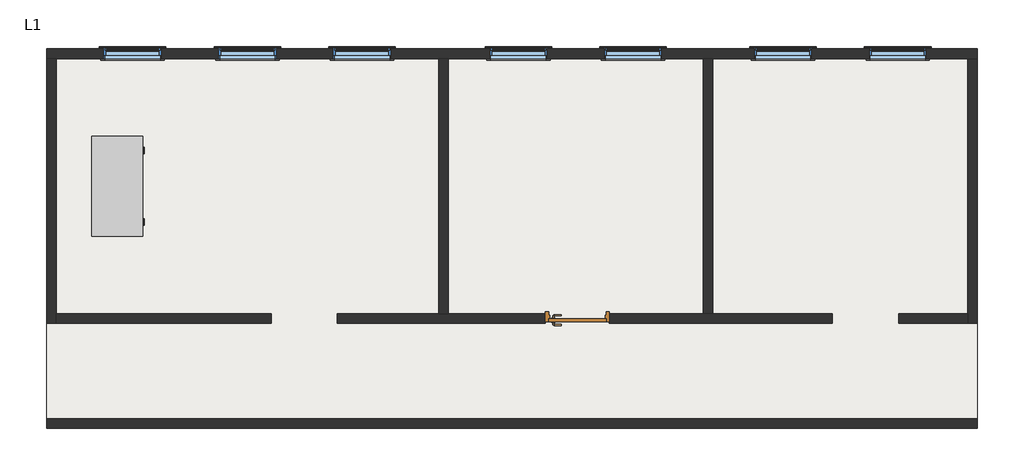
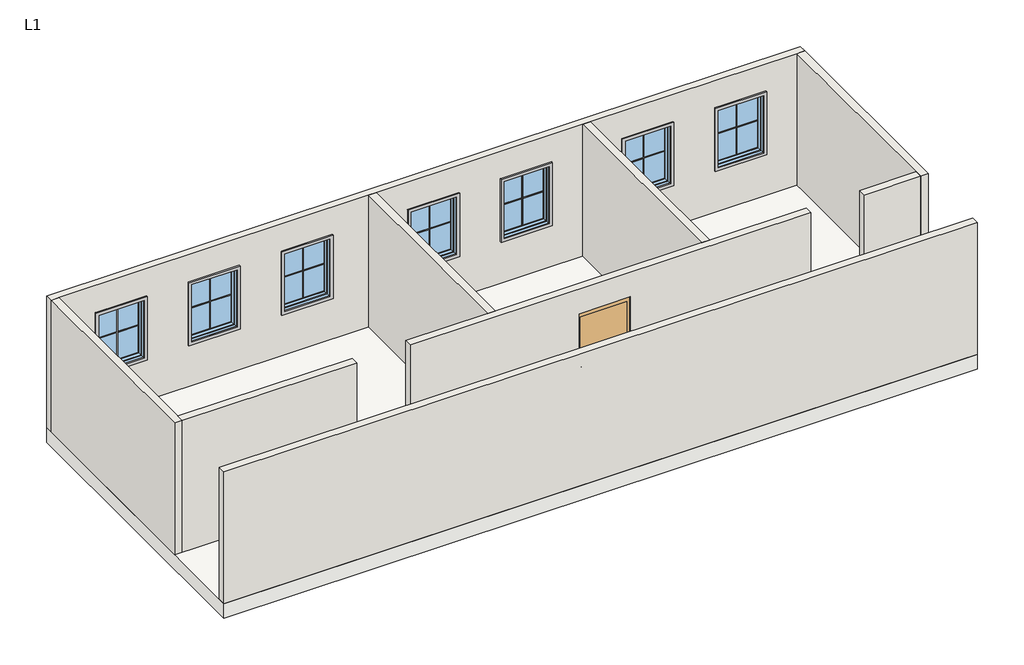
# One storey: 21 proxies, 9 walls, 7 windows, 1 door, 1 furniture element, 1 slab.
"""IFC4 building model written with IfcOpenShell, lengths in millimetres."""

import ifcopenshell
import ifcopenshell.guid

model = None  # the IFC model being written
_history = None  # IfcOwnerHistory: only IFC2X3 demands one
_inside = {}  # id of a spatial element -> (the spatial element, [elements in it])
_under = {}  # id of a project, library or spatial element -> (it, [spatial elements below it])
_declared = {}  # id of a project -> (the project, [libraries it declares])
_typed = {}  # id of a type object -> (the type object, [elements of that type])
_made_of = {}  # id of a material, layer set ... -> (it, [elements and type objects made of it])


def new_model(schema):
    """Start an empty IFC model of exactly this schema.

    Asked for "IFC4X3", IfcOpenShell would pick the latest addendum, in which some entities
    have other attributes; the version numbers below select the first issue.
    IFC2X3 requires an IfcOwnerHistory on every rooted entity: one is made here for all.
    """
    global model, _history
    if schema == "IFC4X3":
        model = ifcopenshell.file(schema_version=(4, 3, 0, 0))
    else:
        model = ifcopenshell.file(schema=schema)
    _inside.clear()
    _under.clear()
    _declared.clear()
    _typed.clear()
    _made_of.clear()
    _history = None
    if model.schema == "IFC2X3":
        org = make("IfcOrganization", Name="unknown")
        user = make(
            "IfcPersonAndOrganization",
            ThePerson=make("IfcPerson", FamilyName="unknown"),
            TheOrganization=org,
        )
        app = make(
            "IfcApplication",
            ApplicationDeveloper=org,
            Version="unknown",
            ApplicationFullName="unknown",
            ApplicationIdentifier="unknown",
        )
        _history = make(
            "IfcOwnerHistory",
            OwningUser=user,
            OwningApplication=app,
            ChangeAction="ADDED",
            CreationDate=0,
        )
    return model


def make(cls, **values):
    """One entity of the class cls with the attributes given. An attribute that is None is left unset."""
    return model.create_entity(
        cls, **{name: value for name, value in values.items() if value is not None}
    )


def rooted(cls, **values):
    """An entity with a GlobalId (a new one), such as an element, a storey or a relation."""
    return make(cls, GlobalId=ifcopenshell.guid.new(), OwnerHistory=_history, **values)


def si_unit(unit_type, name, prefix=None):
    """IfcSIUnit, for example si_unit("LENGTHUNIT", "METRE", prefix="MILLI")."""
    return make("IfcSIUnit", UnitType=unit_type, Prefix=prefix, Name=name)


def assignment(units):
    """IfcUnitAssignment: the units of a project."""
    return None if units is None else make("IfcUnitAssignment", Units=units)


def point(xyz):
    """IfcCartesianPoint."""
    return None if xyz is None else make("IfcCartesianPoint", Coordinates=xyz)


def direction(xyz):
    """IfcDirection."""
    return None if xyz is None else make("IfcDirection", DirectionRatios=xyz)


def frame(location, z_axis=None, x_axis=None):
    """IfcAxis2Placement3D, a coordinate frame: its origin and axes. An axis left out is left unset."""
    return make(
        "IfcAxis2Placement3D",
        Location=point(location),
        Axis=direction(z_axis),
        RefDirection=direction(x_axis),
    )


def frame_2d(location, x_axis=None):
    """IfcAxis2Placement2D, a coordinate frame in the plane: its origin and x axis."""
    return make(
        "IfcAxis2Placement2D", Location=point(location), RefDirection=direction(x_axis)
    )


def origin():
    """The frame at (0, 0, 0) with its axes left unset."""
    return frame((0.0, 0.0, 0.0))


def origin_with_axes():
    """The frame at (0, 0, 0) with the z axis (0, 0, 1) and the x axis (1, 0, 0) written out."""
    return frame((0.0, 0.0, 0.0), z_axis=(0.0, 0.0, 1.0), x_axis=(1.0, 0.0, 0.0))


def place(relative_to, where):
    """IfcLocalPlacement: puts the frame where relative to a parent placement (None: the world)."""
    return make(
        "IfcLocalPlacement", PlacementRelTo=relative_to, RelativePlacement=where
    )


def context(
    kind, dimensions, precision=None, world=None, true_north=None, identifier=None
):
    """IfcGeometricRepresentationContext, for example the 3D "Model" context."""
    return make(
        "IfcGeometricRepresentationContext",
        ContextIdentifier=identifier,
        ContextType=kind,
        CoordinateSpaceDimension=dimensions,
        Precision=precision,
        WorldCoordinateSystem=world,
        TrueNorth=true_north,
    )


def project(units=None, contexts=None):
    """IfcProject with its units and contexts."""
    return rooted(
        "IfcProject",
        Name="project",
        RepresentationContexts=contexts,
        UnitsInContext=assignment(units),
    )


def spatial(cls, under=None, at=None, **own):
    """A site, building, storey or space (cls), placed at a placement, below another one or the project."""
    s = rooted(cls, ObjectPlacement=at, **own)
    if under is not None:
        _under.setdefault(under.id(), (under, []))[1].append(s)
    return s


def polyline(points):
    """IfcPolyline through the points."""
    return make("IfcPolyline", Points=[point(p) for p in points])


def circle_curve(where, radius):
    """IfcCircle in the frame where."""
    return make("IfcCircle", Position=where, Radius=radius)


def ellipse_curve(where, semi_axis1, semi_axis2):
    """IfcEllipse in the frame where."""
    return make(
        "IfcEllipse", Position=where, SemiAxis1=semi_axis1, SemiAxis2=semi_axis2
    )


def trimmed(basis, trim1, trim2, sense, master):
    """IfcTrimmedCurve: the piece of a basis curve between two trims."""
    return make(
        "IfcTrimmedCurve",
        BasisCurve=basis,
        Trim1=trim1,
        Trim2=trim2,
        SenseAgreement=sense,
        MasterRepresentation=master,
    )


def segment(curve, same_sense, transition):
    """IfcCompositeCurveSegment."""
    return make(
        "IfcCompositeCurveSegment",
        Transition=transition,
        SameSense=same_sense,
        ParentCurve=curve,
    )


def composite_curve(segments, self_intersect=None):
    """IfcCompositeCurve: segments joined end to end."""
    return make("IfcCompositeCurve", Segments=segments, SelfIntersect=self_intersect)


def outline(outer, holes=None, kind="AREA"):
    """IfcArbitraryClosedProfileDef: a profile drawn as a closed curve; with holes, ...WithVoids."""
    if holes is None:
        return make("IfcArbitraryClosedProfileDef", ProfileType=kind, OuterCurve=outer)
    return make(
        "IfcArbitraryProfileDefWithVoids",
        ProfileType=kind,
        OuterCurve=outer,
        InnerCurves=holes,
    )


def extrude(swept, where, along, depth):
    """IfcExtrudedAreaSolid: the profile swept, set in the frame where, extruded along a direction by depth."""
    return make(
        "IfcExtrudedAreaSolid",
        SweptArea=swept,
        Position=where,
        ExtrudedDirection=direction(along),
        Depth=depth,
    )


def faces_of(points, faces, orient=None, outer=None):
    """IfcFace entities. A face is a list of loops; a loop is a list of indices into points, from 0.

    orient and outer hold one flag for each loop. By default every Orientation is true, the
    first loop of a face is its IfcFaceOuterBound and the others are IfcFaceBound.
    """
    made = []
    for i, loops in enumerate(faces):
        bounds = []
        for j, loop in enumerate(loops):
            is_outer = j == 0 if outer is None else outer[i][j]
            bounds.append(
                make(
                    "IfcFaceOuterBound" if is_outer else "IfcFaceBound",
                    Bound=make("IfcPolyLoop", Polygon=[points[k] for k in loop]),
                    Orientation=True if orient is None else orient[i][j],
                )
            )
        made.append(make("IfcFace", Bounds=bounds))
    return made


def faceted_brep(points, faces, orient=None, outer=None, voids=None):
    """IfcFacetedBrep: a solid bounded by flat faces; with voids (closed shells), ...WithVoids."""
    shared = [point(p) for p in points]
    hull = make("IfcClosedShell", CfsFaces=faces_of(shared, faces, orient, outer))
    if voids is None:
        return make("IfcFacetedBrep", Outer=hull)
    return make(
        "IfcFacetedBrepWithVoids",
        Outer=hull,
        Voids=[
            make(cls, CfsFaces=faces_of(shared, fs, o, b)) for cls, fs, o, b in voids
        ],
    )


def shape(context_of_items, identifier, shape_type, items):
    """IfcShapeRepresentation: the items that make up one representation, for example the "Body"."""
    return make(
        "IfcShapeRepresentation",
        ContextOfItems=context_of_items,
        RepresentationIdentifier=identifier,
        RepresentationType=shape_type,
        Items=items,
    )


def source(mapping_origin, context_of_items, identifier, shape_type, items):
    """IfcRepresentationMap: a shape defined once, which mapped items show again and again."""
    return make(
        "IfcRepresentationMap",
        MappingOrigin=mapping_origin,
        MappedRepresentation=shape(context_of_items, identifier, shape_type, items),
    )


def transform(
    local_origin,
    x_axis=None,
    y_axis=None,
    z_axis=None,
    scale=None,
    scale2=None,
    scale3=None,
    uniform=True,
):
    """IfcCartesianTransformationOperator3D, or its non-uniform kind. x_axis, y_axis, z_axis: its Axis1, 2, 3."""
    if uniform:
        return make(
            "IfcCartesianTransformationOperator3D",
            Axis1=direction(x_axis),
            Axis2=direction(y_axis),
            LocalOrigin=point(local_origin),
            Scale=scale,
            Axis3=direction(z_axis),
        )
    return make(
        "IfcCartesianTransformationOperator3DnonUniform",
        Axis1=direction(x_axis),
        Axis2=direction(y_axis),
        LocalOrigin=point(local_origin),
        Scale=scale,
        Axis3=direction(z_axis),
        Scale2=scale2,
        Scale3=scale3,
    )


def mapped(mapping_source, mapping_target):
    """IfcMappedItem: shows the shape of a source again, moved by a transform."""
    return make(
        "IfcMappedItem", MappingSource=mapping_source, MappingTarget=mapping_target
    )


def made_of(thing, what):
    """Note that an element or type object is made of a material, layer set ...; save() writes the relation."""
    if what is not None:
        _made_of.setdefault(what.id(), (what, []))[1].append(thing)
    return thing


def element(
    cls,
    number,
    at=None,
    inside=None,
    cuts=None,
    type_object=None,
    material=None,
    context=None,
    identifier="Body",
    shape_type=None,
    held_by="IfcProductDefinitionShape",
    body=None,
    shapes=None,
    **own,
):
    """One element of the class cls, such as IfcWall. Its Tag is "e" and its number.

    at: its placement. inside: the storey or other place that contains it. cuts: it is an
    opening in that element (IfcRelVoidsElement). A single representation is given by context,
    identifier, shape_type and body (its items); several are given by shapes. held_by: the class
    of the entity that holds the representations. save() writes the other relations.
    """
    e = rooted(cls, Tag="e%d" % number, ObjectPlacement=at, **own)
    if body is not None:
        shapes = [shape(context, identifier, shape_type, body)]
    if shapes is not None:
        e.Representation = make(held_by, Representations=shapes)
    if inside is not None:
        _inside.setdefault(inside.id(), (inside, []))[1].append(e)
    if cuts is not None:
        rooted(
            "IfcRelVoidsElement", RelatingBuildingElement=cuts, RelatedOpeningElement=e
        )
    if type_object is not None:
        _typed.setdefault(type_object.id(), (type_object, []))[1].append(e)
    return made_of(e, material)


def aggregate(whole, parts):
    """IfcRelAggregates: a whole, such as a stair, and the parts it consists of."""
    return rooted("IfcRelAggregates", RelatingObject=whole, RelatedObjects=parts)


def save(model, path):
    """Write the relations noted so far, then the file.

    IfcRelAggregates (storeys below a building ...), IfcRelContainedInSpatialStructure (elements
    in a storey), IfcRelDefinesByType, IfcRelAssociatesMaterial and IfcRelDeclares: one each for
    every whole, place, type object, material and project.
    """
    for whole, parts in _under.values():
        aggregate(whole, parts)
    for where, things in _inside.values():
        rooted(
            "IfcRelContainedInSpatialStructure",
            RelatedElements=things,
            RelatingStructure=where,
        )
    for kind, things in _typed.values():
        rooted("IfcRelDefinesByType", RelatedObjects=things, RelatingType=kind)
    for what, things in _made_of.values():
        rooted("IfcRelAssociatesMaterial", RelatedObjects=things, RelatingMaterial=what)
    for by, libraries in _declared.values():
        rooted("IfcRelDeclares", RelatingContext=by, RelatedDefinitions=libraries)
    model.write(path)


def plane_surface(at):
    """IfcPlane: the flat surface through the origin of the frame at, square to its z axis."""
    return make("IfcPlane", Position=at)


def cylinder_surface(at, radius):
    """IfcCylindricalSurface: all points at the distance radius from the z axis of the frame at."""
    return make("IfcCylindricalSurface", Position=at, Radius=radius)


def revolved_surface(curve, axis_point, axis_direction):
    """IfcSurfaceOfRevolution: the curve turned about the line through axis_point along axis_direction."""
    return make(
        "IfcSurfaceOfRevolution",
        SweptCurve=make("IfcArbitraryOpenProfileDef", ProfileType="CURVE", Curve=curve),
        AxisPosition=make("IfcAxis1Placement", Location=point(axis_point), Axis=direction(axis_direction)),
    )


def advanced_brep(points, edges, surfaces, faces):
    """IfcAdvancedBrep: a solid bounded by faces that lie on surfaces and meet in shared edges.

    An edge is (start, end): straight between two places in points (the first is 0);
    or (start, end, curve); or (start, end, curve, False) where it runs against its curve.
    A face is (place in surfaces, loops), or (place, loops, False) where it looks against
    its surface's normal. A loop lists edges by number (the first is 1), with a minus sign
    where the edge is run from its end to its start. The first loop is the outer one.
    """
    corners = [point(p) for p in points]
    vertices = [make("IfcVertexPoint", VertexGeometry=c) for c in corners]
    made = []
    for start, end, *more in edges:
        made.append(
            make(
                "IfcEdgeCurve",
                EdgeStart=vertices[start],
                EdgeEnd=vertices[end],
                EdgeGeometry=more[0] if more else make("IfcPolyline", Points=[corners[start], corners[end]]),
                SameSense=more[1] if len(more) > 1 else True,
            )
        )
    hull = []
    for where, loops, *sense in faces:
        bounds = []
        for j, loop in enumerate(loops):
            ring = [make("IfcOrientedEdge", EdgeElement=made[abs(k) - 1], Orientation=k > 0) for k in loop]
            bounds.append(
                make(
                    "IfcFaceOuterBound" if j == 0 else "IfcFaceBound",
                    Bound=make("IfcEdgeLoop", EdgeList=ring),
                    Orientation=True,
                )
            )
        hull.append(make("IfcAdvancedFace", Bounds=bounds, FaceSurface=surfaces[where], SameSense=sense[0] if sense else True))
    return make("IfcAdvancedBrep", Outer=make("IfcClosedShell", CfsFaces=hull))


def m_muntin_pattern_2x2_m_muntin_pattern_2x2_ad852c99(model_context):
    return source(origin(), model_context, "Body", "SweptSolid", [
        extrude(outline(polyline([(568.25, -6.35), (568.25, -411.9), (555.55, -411.9), (555.55, -6.35), (0.0, -6.35), (0.0, 6.35), (555.55, 6.35), (555.55, 411.9), (568.25, 411.9), (568.25, 6.35), (1123.8, 6.35), (1123.8, -6.35), (568.25, -6.35)])), frame((0.0, -22.225, 0.0), z_axis=(0.0, 1.0, 0.0), x_axis=(0.0, 0.0, 1.0)), (0.0, 0.0, 1.0), 12.7),
        extrude(outline(polyline([(568.25, -6.35), (568.25, -411.9), (555.55, -411.9), (555.55, -6.35), (0.0, -6.35), (0.0, 6.35), (555.55, 6.35), (555.55, 411.9), (568.25, 411.9), (568.25, 6.35), (1123.8, 6.35), (1123.8, -6.35), (568.25, -6.35)])), frame((0.0, 9.525, 0.0), z_axis=(0.0, 1.0, 0.0), x_axis=(0.0, 0.0, 1.0)), (0.0, 0.0, 1.0), 12.7),
    ])


def m_trim_window_exterior_flat_with_sill_71544b40(model_context):
    return source(origin(), model_context, "Body", "SweptSolid", [
        extrude(outline(polyline([(510.0, -1220.4323709), (510.0, -1280.4323709), (-510.0, -1280.4323709), (-510.0, -1220.4323709), (510.0, -1220.4323709)])), origin_with_axes(), (0.0, 0.0, 1.0), 19.05),
        extrude(outline(polyline([(-1230.0, 38.1), (-1202.4580645, 38.1), (-1200.0, 19.05), (-1200.0, 0.0), (-1220.4323709, 0.0), (-1220.4323709, 19.05), (-1230.0, 19.05), (-1230.0, 38.1)])), frame((-522.7, 0.0, 0.0), z_axis=(1.0, 0.0, 0.0), x_axis=(0.0, 1.0, 0.0)), (0.0, 0.0, 1.0), 1045.4),
        extrude(outline(polyline([(-510.0, 60.0), (510.0, 60.0), (510.0, -1200.0), (450.0, -1200.0), (450.0, 0.0), (-450.0, 0.0), (-450.0, -1200.0), (-510.0, -1200.0), (-510.0, 60.0)])), origin_with_axes(), (0.0, 0.0, 1.0), 19.05),
    ])


def m_trim_window_interior_flat_picture_frame_24fe8ef8(model_context):
    return source(origin(), model_context, "Body", "SweptSolid", [
        extrude(outline(polyline([(497.3, 47.3), (497.3, -1247.3), (-497.3, -1247.3), (-497.3, 47.3), (497.3, 47.3)]), holes=[polyline([(437.3, -12.7), (-437.3, -12.7), (-437.3, -1187.3), (437.3, -1187.3), (437.3, -12.7)])]), origin_with_axes(), (0.0, 0.0, 1.0), 30.0),
    ])


def m_door_passage_single_flush_900_x_2100mm_89322b7b(model_context):
    return source(origin(), model_context, "Body", "SolidModel", [
        advanced_brep(
        [(-384.990625, -3.35, 1000.0), (-364.990625, -3.35, 1000.0), (-384.990625, 26.65, 1000.0), (-364.990625, 26.65, 1000.0), (-359.990625, 31.65, 1000.0), (-359.990625, 51.65, 1000.0), (-254.990625, 51.65, 1000.0), (-254.990625, 31.65, 1000.0)],
        [
            (0, 1, circle_curve(frame((-374.990625, -3.35, 1000.0), z_axis=(0.0, -1.0, 0.0), x_axis=(1.0, 0.0, 0.0)), 10.0)),
            (1, 0, circle_curve(frame((-374.990625, -3.35, 1000.0), z_axis=(0.0, -1.0, 0.0), x_axis=(1.0, 0.0, 0.0)), 10.0)),
            (0, 2),
            (2, 3, circle_curve(frame((-374.990625, 26.65, 1000.0), z_axis=(0.0, -1.0, 0.0), x_axis=(1.0, 0.0, 0.0)), 10.0)),
            (3, 1),
            (3, 2, circle_curve(frame((-374.990625, 26.65, 1000.0), z_axis=(0.0, -1.0, 0.0), x_axis=(1.0, 0.0, 0.0)), 10.0)),
            (4, 3, circle_curve(frame((-359.990625, 26.65, 1000.0), z_axis=(0.0, 0.0, 1.0), x_axis=(-1.0, 0.0, 0.0)), 5.0)),
            (2, 5, circle_curve(frame((-359.990625, 26.65, 1000.0), z_axis=(0.0, 0.0, -1.0), x_axis=(-1.0, 0.0, 0.0)), 25.0)),
            (5, 4, circle_curve(frame((-359.990625, 41.65, 1000.0), z_axis=(-1.0, 0.0, 0.0), x_axis=(0.0, -1.0, 0.0)), 10.0)),
            (4, 5, circle_curve(frame((-359.990625, 41.65, 1000.0), z_axis=(-1.0, 0.0, 0.0), x_axis=(0.0, -1.0, 0.0)), 10.0)),
            (6, 7, circle_curve(frame((-254.990625, 41.65, 1000.0), z_axis=(1.0, 0.0, 0.0), x_axis=(0.0, -1.0, 0.0)), 10.0)),
            (7, 6, circle_curve(frame((-254.990625, 41.65, 1000.0), z_axis=(1.0, 0.0, 0.0), x_axis=(0.0, -1.0, 0.0)), 10.0)),
            (5, 6),
            (7, 4),
        ],
        [
            plane_surface(frame((-374.990625, -3.35, 1000.0), z_axis=(0.0, -1.0, 0.0), x_axis=(0.0, 0.0, 1.0))),
            cylinder_surface(frame((-374.990625, -3.35, 1000.0), z_axis=(0.0, -1.0, 0.0), x_axis=(1.0, 0.0, 0.0)), 10.0),
            revolved_surface(trimmed(ellipse_curve(frame((-374.990625, 26.65, 1000.0), z_axis=(0.0, -1.0, 0.0), x_axis=(1.0, 0.0, 0.0)), 10.0, 10.0), [point((-384.990625, 26.65, 1000.0))], [point((-364.990625, 26.65, 1000.0))], True, "CARTESIAN"), (-359.990625, 26.65, 1000.0), (0.0, 0.0, -1.0)),
            revolved_surface(trimmed(ellipse_curve(frame((-374.990625, 26.65, 1000.0), z_axis=(0.0, -1.0, 0.0), x_axis=(1.0, 0.0, 0.0)), 10.0, 10.0), [point((-364.990625, 26.65, 1000.0))], [point((-384.990625, 26.65, 1000.0))], True, "CARTESIAN"), (-359.990625, 26.65, 1000.0), (0.0, 0.0, -1.0)),
            plane_surface(frame((-254.990625, 41.65, 1000.0), z_axis=(1.0, 0.0, 0.0), x_axis=(0.0, 0.0, 1.0))),
            cylinder_surface(frame((-359.990625, 41.65, 1000.0), z_axis=(-1.0, 0.0, 0.0), x_axis=(0.0, -1.0, 0.0)), 10.0),
        ],
        [
            (0, [[1, 2]]),
            (1, [[-1, 3, 4, 5]]),
            (1, [[-2, -5, 6, -3]]),
            (2, [[7, -4, 8, 9]]),
            (3, [[-8, -6, -7, 10]]),
            (4, [[11, 12]]),
            (5, [[-9, 13, -12, 14]]),
            (5, [[-10, -14, -11, -13]]),
        ],
    ),
        extrude(outline(composite_curve([segment(trimmed(circle_curve(frame_2d((1000.0, -377.490625)), 30.0), [point((1000.0, -407.490625))], [point((1000.0, -347.490625))], False, "CARTESIAN"), True, "CONTINUOUS"), segment(trimmed(circle_curve(frame_2d((1000.0, -377.490625)), 30.0), [point((1000.0, -347.490625))], [point((1000.0, -407.490625))], False, "CARTESIAN"), True, "CONTINUOUS")], self_intersect=False)), frame((0.0, -11.35, 0.0), z_axis=(0.0, 1.0, 0.0), x_axis=(0.0, 0.0, 1.0)), (0.0, 0.0, 1.0), 8.0),
        advanced_brep(
        [(-384.990625, -64.35, 1000.0), (-364.990625, -64.35, 1000.0), (-364.990625, -94.35, 1000.0), (-384.990625, -94.35, 1000.0), (-359.990625, -99.35, 1000.0), (-359.990625, -119.35, 1000.0), (-254.990625, -119.35, 1000.0), (-254.990625, -99.35, 1000.0)],
        [
            (0, 1, circle_curve(frame((-374.990625, -64.35, 1000.0), z_axis=(0.0, 1.0, 0.0), x_axis=(1.0, 0.0, 0.0)), 10.0)),
            (1, 0, circle_curve(frame((-374.990625, -64.35, 1000.0), z_axis=(0.0, 1.0, 0.0), x_axis=(1.0, 0.0, 0.0)), 10.0)),
            (1, 2),
            (2, 3, circle_curve(frame((-374.990625, -94.35, 1000.0), z_axis=(0.0, 1.0, 0.0), x_axis=(1.0, 0.0, 0.0)), 10.0)),
            (3, 0),
            (3, 2, circle_curve(frame((-374.990625, -94.35, 1000.0), z_axis=(0.0, 1.0, 0.0), x_axis=(1.0, 0.0, 0.0)), 10.0)),
            (4, 5, circle_curve(frame((-359.990625, -109.35, 1000.0), z_axis=(-1.0, 0.0, 0.0), x_axis=(0.0, 1.0, 0.0)), 10.0)),
            (5, 3, circle_curve(frame((-359.990625, -94.35, 1000.0), z_axis=(0.0, 0.0, -1.0), x_axis=(-1.0, 0.0, 0.0)), 25.0)),
            (2, 4, circle_curve(frame((-359.990625, -94.35, 1000.0), z_axis=(0.0, 0.0, 1.0), x_axis=(-1.0, 0.0, 0.0)), 5.0)),
            (5, 4, circle_curve(frame((-359.990625, -109.35, 1000.0), z_axis=(-1.0, 0.0, 0.0), x_axis=(0.0, 1.0, 0.0)), 10.0)),
            (6, 7, circle_curve(frame((-254.990625, -109.35, 1000.0), z_axis=(1.0, 0.0, 0.0), x_axis=(0.0, 1.0, 0.0)), 10.0)),
            (7, 6, circle_curve(frame((-254.990625, -109.35, 1000.0), z_axis=(1.0, 0.0, 0.0), x_axis=(0.0, 1.0, 0.0)), 10.0)),
            (4, 7),
            (6, 5),
        ],
        [
            plane_surface(frame((-374.990625, -64.35, 1000.0), z_axis=(0.0, 1.0, 0.0), x_axis=(0.0, 0.0, 1.0))),
            cylinder_surface(frame((-374.990625, -64.35, 1000.0), z_axis=(0.0, 1.0, 0.0), x_axis=(1.0, 0.0, 0.0)), 10.0),
            revolved_surface(trimmed(ellipse_curve(frame((-374.990625, -94.35, 1000.0), z_axis=(0.0, -1.0, 0.0), x_axis=(1.0, 0.0, 0.0)), 10.0, 10.0), [point((-384.990625, -94.35, 1000.0))], [point((-364.990625, -94.35, 1000.0))], True, "CARTESIAN"), (-359.990625, -94.35, 1000.0), (0.0, 0.0, -1.0)),
            revolved_surface(trimmed(ellipse_curve(frame((-374.990625, -94.35, 1000.0), z_axis=(0.0, -1.0, 0.0), x_axis=(1.0, 0.0, 0.0)), 10.0, 10.0), [point((-364.990625, -94.35, 1000.0))], [point((-384.990625, -94.35, 1000.0))], True, "CARTESIAN"), (-359.990625, -94.35, 1000.0), (0.0, 0.0, -1.0)),
            plane_surface(frame((-254.990625, -109.35, 1000.0), z_axis=(1.0, 0.0, 0.0), x_axis=(0.0, 0.0, 1.0))),
            cylinder_surface(frame((-359.990625, -109.35, 1000.0), z_axis=(-1.0, 0.0, 0.0), x_axis=(0.0, 1.0, 0.0)), 10.0),
        ],
        [
            (0, [[1, 2]]),
            (1, [[3, 4, 5, -2]]),
            (1, [[-5, 6, -3, -1]]),
            (2, [[7, 8, -4, 9]]),
            (3, [[10, -9, -6, -8]]),
            (4, [[11, 12]]),
            (5, [[13, -11, 14, -7]]),
            (5, [[-14, -12, -13, -10]]),
        ],
    ),
        extrude(outline(composite_curve([segment(trimmed(circle_curve(frame_2d((1000.0, -377.490625)), 30.0), [point((1000.0, -407.490625))], [point((1000.0, -347.490625))], False, "CARTESIAN"), True, "CONTINUOUS"), segment(trimmed(circle_curve(frame_2d((1000.0, -377.490625)), 30.0), [point((1000.0, -347.490625))], [point((1000.0, -407.490625))], False, "CARTESIAN"), True, "CONTINUOUS")], self_intersect=False)), frame((0.0, -64.35, 0.0), z_axis=(0.0, 1.0, 0.0), x_axis=(0.0, 0.0, 1.0)), (0.0, 0.0, 1.0), 8.0),
        extrude(outline(polyline([(450.0, -11.35), (450.0, -56.35), (-450.0, -56.35), (-450.0, -11.35), (450.0, -11.35)])), origin_with_axes(), (0.0, 0.0, 1.0), 2100.0),
        faceted_brep([(450.0, -6.5875, 0.0), (434.125, -6.5875, 0.0), (434.125, 44.4375, 0.0), (450.0, 44.4375, 0.0), (450.0, 93.65, 0.0), (500.0, 93.65, 0.0), (500.0, -56.35, 0.0), (450.0, -56.35, 0.0), (450.0, -56.35, 2100.0), (450.0, -6.5875, 2100.0), (500.0, -56.35, 2200.0), (-500.0, -56.35, 2200.0), (-500.0, -56.35, 0.0), (-450.0, -56.35, 0.0), (-450.0, -56.35, 2100.0), (500.0, 93.65, 2200.0), (450.0, 93.65, 2100.0), (-450.0, 93.65, 2100.0), (-450.0, 93.65, 0.0), (-500.0, 93.65, 0.0), (-500.0, 93.65, 2200.0), (450.0, 44.4375, 2100.0), (434.125, 44.4375, 2084.125), (-434.125, 44.4375, 2084.125), (-434.125, 44.4375, 0.0), (-450.0, 44.4375, 0.0), (-450.0, 44.4375, 2100.0), (434.125, -6.5875, 2084.125), (-450.0, -6.5875, 2100.0), (-450.0, -6.5875, 0.0), (-434.125, -6.5875, 0.0), (-434.125, -6.5875, 2084.125)], [[[0, 1, 2, 3, 4, 5, 6, 7]], [[7, 8, 9, 0]], [[6, 10, 11, 12, 13, 14, 8, 7]], [[5, 15, 10, 6]], [[4, 16, 17, 18, 19, 20, 15, 5]], [[3, 21, 16, 4]], [[2, 22, 23, 24, 25, 26, 21, 3]], [[1, 27, 22, 2]], [[0, 9, 28, 29, 30, 31, 27, 1]], [[8, 14, 28, 9]], [[16, 21, 26, 17]], [[22, 27, 31, 23]], [[12, 19, 18, 25, 24, 30, 29, 13]], [[13, 29, 28, 14]], [[11, 20, 19, 12]], [[17, 26, 25, 18]], [[23, 31, 30, 24]], [[15, 20, 11, 10]]]),
    ])


def m_desk_1525_x_762mm_student_34485ced(model_context):
    return source(origin(), model_context, "Body", "SolidModel", [
        extrude(outline(polyline([(1118.1, 0.0), (1118.1, 635.0), (405.9, 635.0), (405.9, 0.0), (-0.5, 0.0), (-0.5, 762.0), (1524.5, 762.0), (1524.5, 0.0), (1118.1, 0.0)])), frame((0.0, 0.0, 152.0), z_axis=(0.0, 0.0, 1.0), x_axis=(1.0, 0.0, 0.0)), (0.0, 0.0, 1.0), 571.9),
        extrude(outline(polyline([(-19.55, -19.05), (-19.55, 781.05), (1543.55, 781.05), (1543.55, -19.05), (-19.55, -19.05)])), frame((0.0, 0.0, 723.9), z_axis=(0.0, 0.0, 1.0), x_axis=(1.0, 0.0, 0.0)), (0.0, 0.0, 1.0), 38.1),
        faceted_brep([(1422.9, 0.0, 152.0), (1524.5, 0.0, 152.0), (1524.5, 101.6, 152.0), (1422.9, 101.6, 152.0), (1448.3, 0.0, 0.0), (1448.3, 76.2, 0.0), (1524.5, 76.2, 0.0), (1524.5, 0.0, 0.0)], [[[0, 1, 2, 3]], [[4, 5, 6, 7]], [[4, 7, 1, 0]], [[7, 6, 2, 1]], [[6, 5, 3, 2]], [[5, 4, 0, 3]]]),
        faceted_brep([(1422.9, 762.0, 152.0), (1422.9, 660.4, 152.0), (1524.5, 660.4, 152.0), (1524.5, 762.0, 152.0), (1448.3, 762.0, 0.0), (1524.5, 762.0, 0.0), (1524.5, 685.8, 0.0), (1448.3, 685.8, 0.0)], [[[0, 1, 2, 3]], [[4, 5, 6, 7]], [[4, 7, 1, 0]], [[7, 6, 2, 1]], [[6, 5, 3, 2]], [[5, 4, 0, 3]]]),
        faceted_brep([(101.1, 762.0, 152.0), (-0.5, 762.0, 152.0), (-0.5, 660.4, 152.0), (101.1, 660.4, 152.0), (75.7, 762.0, 0.0), (75.7, 685.8, 0.0), (-0.5, 685.8, 0.0), (-0.5, 762.0, 0.0)], [[[0, 1, 2, 3]], [[4, 5, 6, 7]], [[4, 7, 1, 0]], [[7, 6, 2, 1]], [[6, 5, 3, 2]], [[5, 4, 0, 3]]]),
        faceted_brep([(101.1, 0.0, 152.0), (101.1, 101.6, 152.0), (-0.5, 101.6, 152.0), (-0.5, 0.0, 152.0), (75.7, 0.0, 0.0), (-0.5, 0.0, 0.0), (-0.5, 76.2, 0.0), (75.7, 76.2, 0.0)], [[[0, 1, 2, 3]], [[4, 5, 6, 7]], [[4, 7, 1, 0]], [[7, 6, 2, 1]], [[6, 5, 3, 2]], [[5, 4, 0, 3]]]),
        extrude(outline(polyline([(1137.15, 0.0), (1505.45, 0.0), (1505.45, -12.7), (1137.15, -12.7), (1137.15, 0.0)])), frame((0.0, 0.0, 602.85), z_axis=(0.0, 0.0, 1.0), x_axis=(1.0, 0.0, 0.0)), (0.0, 0.0, 1.0), 102.0),
        extrude(outline(polyline([(1137.15, 0.0), (1505.45, 0.0), (1505.45, -12.7), (1137.15, -12.7), (1137.15, 0.0)])), frame((0.0, 0.0, 171.05), z_axis=(0.0, 0.0, 1.0), x_axis=(1.0, 0.0, 0.0)), (0.0, 0.0, 1.0), 171.45),
        extrude(outline(polyline([(1137.15, 0.0), (1505.45, 0.0), (1505.45, -12.7), (1137.15, -12.7), (1137.15, 0.0)])), frame((0.0, 0.0, 482.2), z_axis=(0.0, 0.0, 1.0), x_axis=(1.0, 0.0, 0.0)), (0.0, 0.0, 1.0), 101.6),
        extrude(outline(polyline([(1137.15, 0.0), (1505.45, 0.0), (1505.45, -12.7), (1137.15, -12.7), (1137.15, 0.0)])), frame((0.0, 0.0, 361.55), z_axis=(0.0, 0.0, 1.0), x_axis=(1.0, 0.0, 0.0)), (0.0, 0.0, 1.0), 101.6),
        extrude(outline(polyline([(18.55, 0.0), (386.85, 0.0), (386.85, -12.7), (18.55, -12.7), (18.55, 0.0)])), frame((0.0, 0.0, 603.25), z_axis=(0.0, 0.0, 1.0), x_axis=(1.0, 0.0, 0.0)), (0.0, 0.0, 1.0), 101.6),
        extrude(outline(polyline([(18.55, 0.0), (386.85, 0.0), (386.85, -12.7), (18.55, -12.7), (18.55, 0.0)])), frame((0.0, 0.0, 171.05), z_axis=(0.0, 0.0, 1.0), x_axis=(1.0, 0.0, 0.0)), (0.0, 0.0, 1.0), 413.15),
        faceted_brep([(1365.75, -12.7, 304.8), (1372.1, -12.7, 304.8), (1372.1, -12.7, 292.1), (1365.75, -12.7, 292.1), (1365.75, -31.75, 304.8), (1372.1, -38.1, 304.8), (1372.1, -38.1, 292.1), (1365.75, -31.75, 292.1), (1276.85, -31.75, 304.8), (1270.5, -38.1, 304.8), (1270.5, -38.1, 292.1), (1276.85, -31.75, 292.1), (1276.85, -12.7, 304.8), (1276.85, -12.7, 292.1), (1270.5, -12.7, 292.1), (1270.5, -12.7, 304.8)], [[[0, 1, 2, 3]], [[1, 0, 4, 5]], [[2, 1, 5, 6]], [[3, 2, 6, 7]], [[0, 3, 7, 4]], [[5, 4, 8, 9]], [[6, 5, 9, 10]], [[7, 6, 10, 11]], [[4, 7, 11, 8]], [[12, 13, 14, 15]], [[9, 8, 12, 15]], [[10, 9, 15, 14]], [[11, 10, 14, 13]], [[8, 11, 13, 12]]]),
        faceted_brep([(1365.75, -12.7, 425.45), (1372.1, -12.7, 425.45), (1372.1, -12.7, 412.75), (1365.75, -12.7, 412.75), (1365.75, -31.75, 425.45), (1372.1, -38.1, 425.45), (1372.1, -38.1, 412.75), (1365.75, -31.75, 412.75), (1276.85, -31.75, 425.45), (1270.5, -38.1, 425.45), (1270.5, -38.1, 412.75), (1276.85, -31.75, 412.75), (1276.85, -12.7, 425.45), (1276.85, -12.7, 412.75), (1270.5, -12.7, 412.75), (1270.5, -12.7, 425.45)], [[[0, 1, 2, 3]], [[1, 0, 4, 5]], [[2, 1, 5, 6]], [[3, 2, 6, 7]], [[0, 3, 7, 4]], [[5, 4, 8, 9]], [[6, 5, 9, 10]], [[7, 6, 10, 11]], [[4, 7, 11, 8]], [[12, 13, 14, 15]], [[9, 8, 12, 15]], [[10, 9, 15, 14]], [[11, 10, 14, 13]], [[8, 11, 13, 12]]]),
        faceted_brep([(1365.75, -12.7, 546.1), (1372.1, -12.7, 546.1), (1372.1, -12.7, 533.4), (1365.75, -12.7, 533.4), (1365.75, -31.75, 546.1), (1372.1, -38.1, 546.1), (1372.1, -38.1, 533.4), (1365.75, -31.75, 533.4), (1276.85, -31.75, 546.1), (1270.5, -38.1, 546.1), (1270.5, -38.1, 533.4), (1276.85, -31.75, 533.4), (1276.85, -12.7, 546.1), (1276.85, -12.7, 533.4), (1270.5, -12.7, 533.4), (1270.5, -12.7, 546.1)], [[[0, 1, 2, 3]], [[1, 0, 4, 5]], [[2, 1, 5, 6]], [[3, 2, 6, 7]], [[0, 3, 7, 4]], [[5, 4, 8, 9]], [[6, 5, 9, 10]], [[7, 6, 10, 11]], [[4, 7, 11, 8]], [[12, 13, 14, 15]], [[9, 8, 12, 15]], [[10, 9, 15, 14]], [[11, 10, 14, 13]], [[8, 11, 13, 12]]]),
        faceted_brep([(1365.75, -12.7, 666.75), (1372.1, -12.7, 666.75), (1372.1, -12.7, 654.05), (1365.75, -12.7, 654.05), (1365.75, -31.75, 666.75), (1372.1, -38.1, 666.75), (1372.1, -38.1, 654.05), (1365.75, -31.75, 654.05), (1276.85, -31.75, 666.75), (1270.5, -38.1, 666.75), (1270.5, -38.1, 654.05), (1276.85, -31.75, 654.05), (1276.85, -12.7, 666.75), (1276.85, -12.7, 654.05), (1270.5, -12.7, 654.05), (1270.5, -12.7, 666.75)], [[[0, 1, 2, 3]], [[1, 0, 4, 5]], [[2, 1, 5, 6]], [[3, 2, 6, 7]], [[0, 3, 7, 4]], [[5, 4, 8, 9]], [[6, 5, 9, 10]], [[7, 6, 10, 11]], [[4, 7, 11, 8]], [[12, 13, 14, 15]], [[9, 8, 12, 15]], [[10, 9, 15, 14]], [[11, 10, 14, 13]], [[8, 11, 13, 12]]]),
        faceted_brep([(158.25, -12.7, 546.1), (158.25, -12.7, 533.4), (151.9, -12.7, 533.4), (151.9, -12.7, 546.1), (158.25, -31.75, 546.1), (158.25, -31.75, 533.4), (151.9, -38.1, 533.4), (151.9, -38.1, 546.1), (247.15, -31.75, 546.1), (247.15, -31.75, 533.4), (253.5, -38.1, 533.4), (253.5, -38.1, 546.1), (247.15, -12.7, 546.1), (253.5, -12.7, 546.1), (253.5, -12.7, 533.4), (247.15, -12.7, 533.4)], [[[0, 1, 2, 3]], [[1, 0, 4, 5]], [[2, 1, 5, 6]], [[3, 2, 6, 7]], [[0, 3, 7, 4]], [[5, 4, 8, 9]], [[6, 5, 9, 10]], [[7, 6, 10, 11]], [[4, 7, 11, 8]], [[12, 13, 14, 15]], [[9, 8, 12, 15]], [[10, 9, 15, 14]], [[11, 10, 14, 13]], [[8, 11, 13, 12]]]),
        faceted_brep([(158.25, -12.7, 666.75), (158.25, -12.7, 654.05), (151.9, -12.7, 654.05), (151.9, -12.7, 666.75), (158.25, -31.75, 666.75), (158.25, -31.75, 654.05), (151.9, -38.1, 654.05), (151.9, -38.1, 666.75), (247.15, -31.75, 666.75), (247.15, -31.75, 654.05), (253.5, -38.1, 654.05), (253.5, -38.1, 666.75), (247.15, -12.7, 666.75), (253.5, -12.7, 666.75), (253.5, -12.7, 654.05), (247.15, -12.7, 654.05)], [[[0, 1, 2, 3]], [[1, 0, 4, 5]], [[2, 1, 5, 6]], [[3, 2, 6, 7]], [[0, 3, 7, 4]], [[5, 4, 8, 9]], [[6, 5, 9, 10]], [[7, 6, 10, 11]], [[4, 7, 11, 8]], [[12, 13, 14, 15]], [[9, 8, 12, 15]], [[10, 9, 15, 14]], [[11, 10, 14, 13]], [[8, 11, 13, 12]]]),
    ])


def m_window_fixed_900_x_1200mm_f2c8dc95(model_context):
    return source(origin(), model_context, "Body", "SolidModel", [
        faceted_brep([(450.0, -20.25, 2100.0), (450.0, 94.05, 2100.0), (-450.0, 94.05, 2100.0), (-450.0, -20.25, 2100.0), (-450.0, 94.05, 900.0), (-450.0, -20.25, 900.0), (450.0, 94.05, 900.0), (450.0, -20.25, 900.0), (418.25, -20.25, 2068.25), (418.25, -20.25, 931.75), (-418.25, -20.25, 931.75), (-418.25, -20.25, 2068.25), (-437.3, 94.05, 2087.3), (-437.3, 94.05, 912.7), (437.3, 94.05, 912.7), (437.3, 94.05, 2087.3), (418.25, 43.25, 2068.25), (-418.25, 43.25, 2068.25), (437.3, 43.25, 2087.3), (-437.3, 43.25, 2087.3), (-418.25, 43.25, 931.75), (-437.3, 43.25, 912.7), (418.25, 43.25, 931.75), (437.3, 43.25, 912.7)], [[[0, 1, 2, 3]], [[3, 2, 4, 5]], [[5, 4, 6, 7]], [[3, 5, 7, 0], [8, 9, 10, 11]], [[7, 6, 1, 0]], [[1, 6, 4, 2], [12, 13, 14, 15]], [[16, 8, 11, 17]], [[15, 18, 19, 12]], [[17, 11, 10, 20]], [[12, 19, 21, 13]], [[20, 10, 9, 22]], [[13, 21, 23, 14]], [[22, 9, 8, 16]], [[18, 23, 21, 19], [17, 20, 22, 16]], [[14, 23, 18, 15]]]),
        extrude(outline(polyline([(2100.0, -450.0), (900.0, -450.0), (900.0, 450.0), (2100.0, 450.0), (2100.0, -450.0)]), holes=[polyline([(2087.3, 437.3), (912.7, 437.3), (912.7, -437.3), (2087.3, -437.3), (2087.3, 437.3)])]), frame((0.0, -75.0, 0.0), z_axis=(0.0, 1.0, 0.0), x_axis=(0.0, 0.0, 1.0)), (0.0, 0.0, 1.0), 54.75),
        extrude(outline(polyline([(912.7, 437.3), (2087.3, 437.3), (2087.3, -437.3), (912.7, -437.3), (912.7, 437.3)]), holes=[polyline([(938.1, -411.9), (2061.9, -411.9), (2061.9, 411.9), (938.1, 411.9), (938.1, -411.9)])]), frame((0.0, 43.25, 0.0), z_axis=(0.0, 1.0, 0.0), x_axis=(0.0, 0.0, 1.0)), (0.0, 0.0, 1.0), 44.45),
        extrude(outline(polyline([(411.9, 75.0), (411.9, 68.65), (-411.9, 68.65), (-411.9, 75.0), (411.9, 75.0)])), frame((0.0, 0.0, 938.1), z_axis=(0.0, 0.0, 1.0), x_axis=(1.0, 0.0, 0.0)), (0.0, 0.0, 1.0), 1123.8),
        extrude(outline(polyline([(-411.9, 55.95), (-411.9, 62.3), (411.9, 62.3), (411.9, 55.95), (-411.9, 55.95)])), frame((0.0, 0.0, 938.1), z_axis=(0.0, 0.0, 1.0), x_axis=(1.0, 0.0, 0.0)), (0.0, 0.0, 1.0), 1123.8),
    ])


model = new_model("IFC4")

# Units and contexts
model_context = context("Model", 3, world=origin())
ifc_project = project(units=[si_unit("LENGTHUNIT", "METRE", prefix="MILLI")], contexts=[model_context])

# Site, building, storey
site = spatial("IfcSite", under=ifc_project)
building = spatial("IfcBuilding", under=site)
storey = spatial("IfcBuildingStorey", under=building, Name="L1", Elevation=0.0)

# Proxies
placement = place(None, origin())
m_muntin_pattern_2x2_m_muntin_pattern_2x2_shape = m_muntin_pattern_2x2_m_muntin_pattern_2x2_ad852c99(model_context)
element("IfcBuildingElementProxy", 1, Name="M_Muntin Pattern_2x2 : M_Muntin Pattern_2x2", ObjectType="M_Muntin Pattern_2x2 : M_Muntin Pattern_2x2", at=placement, inside=storey, context=model_context, shape_type="MappedRepresentation", body=[
    mapped(m_muntin_pattern_2x2_m_muntin_pattern_2x2_shape, transform((2825.0, 4215.475, 938.1), x_axis=(-1.0, 0.0, 0.0), y_axis=(0.0, -1.0, 0.0), z_axis=(0.0, 0.0, 1.0))),
])
element("IfcBuildingElementProxy", 2, Name="M_Muntin Pattern_2x2 : M_Muntin Pattern_2x2", ObjectType="M_Muntin Pattern_2x2 : M_Muntin Pattern_2x2", at=placement, inside=storey, context=model_context, shape_type="MappedRepresentation", body=[
    mapped(m_muntin_pattern_2x2_m_muntin_pattern_2x2_shape, transform((1025.0, 4215.475, 938.1), x_axis=(-1.0, 0.0, 0.0), y_axis=(0.0, -1.0, 0.0), z_axis=(0.0, 0.0, 1.0))),
])
element("IfcBuildingElementProxy", 3, Name="M_Muntin Pattern_2x2 : M_Muntin Pattern_2x2", ObjectType="M_Muntin Pattern_2x2 : M_Muntin Pattern_2x2", at=placement, inside=storey, context=model_context, shape_type="MappedRepresentation", body=[
    mapped(m_muntin_pattern_2x2_m_muntin_pattern_2x2_shape, transform((-1425.0, 4215.475, 938.1), x_axis=(-1.0, 0.0, 0.0), y_axis=(0.0, -1.0, 0.0), z_axis=(0.0, 0.0, 1.0))),
])
element("IfcBuildingElementProxy", 4, Name="M_Muntin Pattern_2x2 : M_Muntin Pattern_2x2", ObjectType="M_Muntin Pattern_2x2 : M_Muntin Pattern_2x2", at=placement, inside=storey, context=model_context, shape_type="MappedRepresentation", body=[
    mapped(m_muntin_pattern_2x2_m_muntin_pattern_2x2_shape, transform((-3225.0, 4215.475, 938.1), x_axis=(-1.0, 0.0, 0.0), y_axis=(0.0, -1.0, 0.0), z_axis=(0.0, 0.0, 1.0))),
])
element("IfcBuildingElementProxy", 5, Name="M_Muntin Pattern_2x2 : M_Muntin Pattern_2x2", ObjectType="M_Muntin Pattern_2x2 : M_Muntin Pattern_2x2", at=placement, inside=storey, context=model_context, shape_type="MappedRepresentation", body=[
    mapped(m_muntin_pattern_2x2_m_muntin_pattern_2x2_shape, transform((-5025.0, 4215.475, 938.1), x_axis=(-1.0, 0.0, 0.0), y_axis=(0.0, -1.0, 0.0), z_axis=(0.0, 0.0, 1.0))),
])
element("IfcBuildingElementProxy", 6, Name="M_Muntin Pattern_2x2 : M_Muntin Pattern_2x2", ObjectType="M_Muntin Pattern_2x2 : M_Muntin Pattern_2x2", at=placement, inside=storey, context=model_context, shape_type="MappedRepresentation", body=[
    mapped(m_muntin_pattern_2x2_m_muntin_pattern_2x2_shape, transform((5175.0, 4215.475, 938.1), x_axis=(-1.0, 0.0, 0.0), y_axis=(0.0, -1.0, 0.0), z_axis=(0.0, 0.0, 1.0))),
])
element("IfcBuildingElementProxy", 7, Name="M_Muntin Pattern_2x2 : M_Muntin Pattern_2x2", ObjectType="M_Muntin Pattern_2x2 : M_Muntin Pattern_2x2", at=placement, inside=storey, context=model_context, shape_type="MappedRepresentation", body=[
    mapped(m_muntin_pattern_2x2_m_muntin_pattern_2x2_shape, transform((6975.0, 4215.475, 938.1), x_axis=(-1.0, 0.0, 0.0), y_axis=(0.0, -1.0, 0.0), z_axis=(0.0, 0.0, 1.0))),
])
m_trim_window_exterior_flat_with_sill_shape = m_trim_window_exterior_flat_with_sill_71544b40(model_context)
element("IfcBuildingElementProxy", 8, Name="M_Trim-Window-Exterior-Flat : with Sill", ObjectType="M_Trim-Window-Exterior-Flat : with Sill", at=placement, inside=storey, context=model_context, shape_type="MappedRepresentation", body=[
    mapped(m_trim_window_exterior_flat_with_sill_shape, transform((2825.0, 4225.0, 2100.0), x_axis=(-1.0, 0.0, 0.0), y_axis=(0.0, 0.0, 1.0), z_axis=(0.0, 1.0, 0.0))),
])
element("IfcBuildingElementProxy", 9, Name="M_Trim-Window-Exterior-Flat : with Sill", ObjectType="M_Trim-Window-Exterior-Flat : with Sill", at=placement, inside=storey, context=model_context, shape_type="MappedRepresentation", body=[
    mapped(m_trim_window_exterior_flat_with_sill_shape, transform((1025.0, 4225.0, 2100.0), x_axis=(-1.0, 0.0, 0.0), y_axis=(0.0, 0.0, 1.0), z_axis=(0.0, 1.0, 0.0))),
])
element("IfcBuildingElementProxy", 10, Name="M_Trim-Window-Exterior-Flat : with Sill", ObjectType="M_Trim-Window-Exterior-Flat : with Sill", at=placement, inside=storey, context=model_context, shape_type="MappedRepresentation", body=[
    mapped(m_trim_window_exterior_flat_with_sill_shape, transform((-1425.0, 4225.0, 2100.0), x_axis=(-1.0, 0.0, 0.0), y_axis=(0.0, 0.0, 1.0), z_axis=(0.0, 1.0, 0.0))),
])
element("IfcBuildingElementProxy", 11, Name="M_Trim-Window-Exterior-Flat : with Sill", ObjectType="M_Trim-Window-Exterior-Flat : with Sill", at=placement, inside=storey, context=model_context, shape_type="MappedRepresentation", body=[
    mapped(m_trim_window_exterior_flat_with_sill_shape, transform((-3225.0, 4225.0, 2100.0), x_axis=(-1.0, 0.0, 0.0), y_axis=(0.0, 0.0, 1.0), z_axis=(0.0, 1.0, 0.0))),
])
element("IfcBuildingElementProxy", 12, Name="M_Trim-Window-Exterior-Flat : with Sill", ObjectType="M_Trim-Window-Exterior-Flat : with Sill", at=placement, inside=storey, context=model_context, shape_type="MappedRepresentation", body=[
    mapped(m_trim_window_exterior_flat_with_sill_shape, transform((-5025.0, 4225.0, 2100.0), x_axis=(-1.0, 0.0, 0.0), y_axis=(0.0, 0.0, 1.0), z_axis=(0.0, 1.0, 0.0))),
])
element("IfcBuildingElementProxy", 13, Name="M_Trim-Window-Exterior-Flat : with Sill", ObjectType="M_Trim-Window-Exterior-Flat : with Sill", at=placement, inside=storey, context=model_context, shape_type="MappedRepresentation", body=[
    mapped(m_trim_window_exterior_flat_with_sill_shape, transform((5175.0, 4225.0, 2100.0), x_axis=(-1.0, 0.0, 0.0), y_axis=(0.0, 0.0, 1.0), z_axis=(0.0, 1.0, 0.0))),
])
element("IfcBuildingElementProxy", 14, Name="M_Trim-Window-Exterior-Flat : with Sill", ObjectType="M_Trim-Window-Exterior-Flat : with Sill", at=placement, inside=storey, context=model_context, shape_type="MappedRepresentation", body=[
    mapped(m_trim_window_exterior_flat_with_sill_shape, transform((6975.0, 4225.0, 2100.0), x_axis=(-1.0, 0.0, 0.0), y_axis=(0.0, 0.0, 1.0), z_axis=(0.0, 1.0, 0.0))),
])
m_trim_window_interior_flat_picture_frame_shape = m_trim_window_interior_flat_picture_frame_24fe8ef8(model_context)
element("IfcBuildingElementProxy", 15, Name="M_Trim-Window-Interior-Flat : Picture Frame", ObjectType="M_Trim-Window-Interior-Flat : Picture Frame", at=placement, inside=storey, context=model_context, shape_type="MappedRepresentation", body=[
    mapped(m_trim_window_interior_flat_picture_frame_shape, transform((2825.0, 4075.0, 2100.0), x_axis=(1.0, 0.0, 0.0), y_axis=(0.0, 0.0, 1.0), z_axis=(0.0, -1.0, 0.0))),
])
element("IfcBuildingElementProxy", 16, Name="M_Trim-Window-Interior-Flat : Picture Frame", ObjectType="M_Trim-Window-Interior-Flat : Picture Frame", at=placement, inside=storey, context=model_context, shape_type="MappedRepresentation", body=[
    mapped(m_trim_window_interior_flat_picture_frame_shape, transform((1025.0, 4075.0, 2100.0), x_axis=(1.0, 0.0, 0.0), y_axis=(0.0, 0.0, 1.0), z_axis=(0.0, -1.0, 0.0))),
])
element("IfcBuildingElementProxy", 17, Name="M_Trim-Window-Interior-Flat : Picture Frame", ObjectType="M_Trim-Window-Interior-Flat : Picture Frame", at=placement, inside=storey, context=model_context, shape_type="MappedRepresentation", body=[
    mapped(m_trim_window_interior_flat_picture_frame_shape, transform((-1425.0, 4075.0, 2100.0), x_axis=(1.0, 0.0, 0.0), y_axis=(0.0, 0.0, 1.0), z_axis=(0.0, -1.0, 0.0))),
])
element("IfcBuildingElementProxy", 18, Name="M_Trim-Window-Interior-Flat : Picture Frame", ObjectType="M_Trim-Window-Interior-Flat : Picture Frame", at=placement, inside=storey, context=model_context, shape_type="MappedRepresentation", body=[
    mapped(m_trim_window_interior_flat_picture_frame_shape, transform((-3225.0, 4075.0, 2100.0), x_axis=(1.0, 0.0, 0.0), y_axis=(0.0, 0.0, 1.0), z_axis=(0.0, -1.0, 0.0))),
])
element("IfcBuildingElementProxy", 19, Name="M_Trim-Window-Interior-Flat : Picture Frame", ObjectType="M_Trim-Window-Interior-Flat : Picture Frame", at=placement, inside=storey, context=model_context, shape_type="MappedRepresentation", body=[
    mapped(m_trim_window_interior_flat_picture_frame_shape, transform((-5025.0, 4075.0, 2100.0), x_axis=(1.0, 0.0, 0.0), y_axis=(0.0, 0.0, 1.0), z_axis=(0.0, -1.0, 0.0))),
])
element("IfcBuildingElementProxy", 20, Name="M_Trim-Window-Interior-Flat : Picture Frame", ObjectType="M_Trim-Window-Interior-Flat : Picture Frame", at=placement, inside=storey, context=model_context, shape_type="MappedRepresentation", body=[
    mapped(m_trim_window_interior_flat_picture_frame_shape, transform((5175.0, 4075.0, 2100.0), x_axis=(1.0, 0.0, 0.0), y_axis=(0.0, 0.0, 1.0), z_axis=(0.0, -1.0, 0.0))),
])
element("IfcBuildingElementProxy", 21, Name="M_Trim-Window-Interior-Flat : Picture Frame", ObjectType="M_Trim-Window-Interior-Flat : Picture Frame", at=placement, inside=storey, context=model_context, shape_type="MappedRepresentation", body=[
    mapped(m_trim_window_interior_flat_picture_frame_shape, transform((6975.0, 4075.0, 2100.0), x_axis=(1.0, 0.0, 0.0), y_axis=(0.0, 0.0, 1.0), z_axis=(0.0, -1.0, 0.0))),
])

# Door
m_door_passage_single_flush_900_x_2100mm_shape = m_door_passage_single_flush_900_x_2100mm_89322b7b(model_context)
element("IfcDoor", 22, ObjectType="M_Door-Passage-Single-Flush : 900 x 2100mm", at=placement, inside=storey, context=model_context, shape_type="MappedRepresentation", body=[
    mapped(m_door_passage_single_flush_900_x_2100mm_shape, transform((1950.0, 6.35, 0.0), x_axis=(1.0, 0.0, 0.0), y_axis=(0.0, 1.0, 0.0), z_axis=(0.0, 0.0, 1.0))),
])

# Furniture
m_desk_1525_x_762mm_student_shape = m_desk_1525_x_762mm_student_34485ced(model_context)
element("IfcFurniture", 23, ObjectType="M_Desk : 1525 x 762mm Student", at=placement, inside=storey, context=model_context, shape_type="MappedRepresentation", body=[
    mapped(m_desk_1525_x_762mm_student_shape, transform((-4883.0, 1310.5, 0.0), x_axis=(0.0, 1.0, 0.0), y_axis=(-1.0, 0.0, 0.0), z_axis=(0.0, 0.0, 1.0))),
])

# Slab
element("IfcSlab", 24, ObjectType="Generic 300mm", at=placement, inside=storey, context=model_context, shape_type="SweptSolid", body=[
    extrude(outline(polyline([(8225.0, 4225.0), (8225.0, -1725.0), (-6375.0, -1725.0), (-6375.0, 4225.0), (8225.0, 4225.0)])), frame((0.0, 0.0, -300.0), z_axis=(0.0, 0.0, 1.0), x_axis=(1.0, 0.0, 0.0)), (0.0, 0.0, 1.0), 300.0),
])

# Walls
element("IfcWall", 25, ObjectType="Generic - 150mm", at=placement, inside=storey, context=model_context, shape_type="SweptSolid", body=[
    extrude(outline(polyline([(-75.0, 4075.0), (-75.0, 75.0), (-225.0, 75.0), (-225.0, 4075.0), (-75.0, 4075.0)])), origin_with_axes(), (0.0, 0.0, 1.0), 2700.0),
])
element("IfcWall", 26, ObjectType="Generic - 150mm", at=placement, inside=storey, context=model_context, shape_type="Brep", body=[
    faceted_brep([(-6375.0, 4075.0, 0.0), (-6225.0, 4075.0, 0.0), (-225.0, 4075.0, 0.0), (-75.0, 4075.0, 0.0), (3925.0, 4075.0, 0.0), (4075.0, 4075.0, 0.0), (8075.0, 4075.0, 0.0), (8225.0, 4075.0, 0.0), (8225.0, 4075.0, 2700.0), (8075.0, 4075.0, 2700.0), (4075.0, 4075.0, 2700.0), (3925.0, 4075.0, 2700.0), (-75.0, 4075.0, 2700.0), (-225.0, 4075.0, 2700.0), (-6225.0, 4075.0, 2700.0), (-6375.0, 4075.0, 2700.0), (3275.0, 4075.0, 2100.0), (3275.0, 4075.0, 900.0), (2375.0, 4075.0, 900.0), (2375.0, 4075.0, 2100.0), (1475.0, 4075.0, 2100.0), (1475.0, 4075.0, 900.0), (575.0, 4075.0, 900.0), (575.0, 4075.0, 2100.0), (-975.0, 4075.0, 2100.0), (-975.0, 4075.0, 900.0), (-1875.0, 4075.0, 900.0), (-1875.0, 4075.0, 2100.0), (-2775.0, 4075.0, 2100.0), (-2775.0, 4075.0, 900.0), (-3675.0, 4075.0, 900.0), (-3675.0, 4075.0, 2100.0), (-4575.0, 4075.0, 2100.0), (-4575.0, 4075.0, 900.0), (-5475.0, 4075.0, 900.0), (-5475.0, 4075.0, 2100.0), (5625.0, 4075.0, 2100.0), (5625.0, 4075.0, 900.0), (4725.0, 4075.0, 900.0), (4725.0, 4075.0, 2100.0), (7425.0, 4075.0, 2100.0), (7425.0, 4075.0, 900.0), (6525.0, 4075.0, 900.0), (6525.0, 4075.0, 2100.0), (-6375.0, 4225.0, 0.0), (-6375.0, 4225.0, 2700.0), (8225.0, 4225.0, 2700.0), (8225.0, 4225.0, 0.0), (3275.0, 4225.0, 2100.0), (2375.0, 4225.0, 2100.0), (2375.0, 4225.0, 900.0), (3275.0, 4225.0, 900.0), (1475.0, 4225.0, 2100.0), (575.0, 4225.0, 2100.0), (575.0, 4225.0, 900.0), (1475.0, 4225.0, 900.0), (-975.0, 4225.0, 2100.0), (-1875.0, 4225.0, 2100.0), (-1875.0, 4225.0, 900.0), (-975.0, 4225.0, 900.0), (-2775.0, 4225.0, 2100.0), (-3675.0, 4225.0, 2100.0), (-3675.0, 4225.0, 900.0), (-2775.0, 4225.0, 900.0), (-4575.0, 4225.0, 2100.0), (-5475.0, 4225.0, 2100.0), (-5475.0, 4225.0, 900.0), (-4575.0, 4225.0, 900.0), (5625.0, 4225.0, 2100.0), (4725.0, 4225.0, 2100.0), (4725.0, 4225.0, 900.0), (5625.0, 4225.0, 900.0), (7425.0, 4225.0, 2100.0), (6525.0, 4225.0, 2100.0), (6525.0, 4225.0, 900.0), (7425.0, 4225.0, 900.0)], [[[0, 1, 2, 3, 4, 5, 6, 7, 8, 9, 10, 11, 12, 13, 14, 15], [16, 17, 18, 19], [20, 21, 22, 23], [24, 25, 26, 27], [28, 29, 30, 31], [32, 33, 34, 35], [36, 37, 38, 39], [40, 41, 42, 43]], [[44, 45, 46, 47], [48, 49, 50, 51], [52, 53, 54, 55], [56, 57, 58, 59], [60, 61, 62, 63], [64, 65, 66, 67], [68, 69, 70, 71], [72, 73, 74, 75]], [[7, 6, 5, 4, 3, 2, 1, 0, 44, 47]], [[15, 14, 13, 12, 11, 10, 9, 8, 46, 45]], [[0, 15, 45, 44]], [[8, 7, 47, 46]], [[17, 16, 48, 51]], [[18, 17, 51, 50]], [[19, 18, 50, 49]], [[16, 19, 49, 48]], [[21, 20, 52, 55]], [[22, 21, 55, 54]], [[23, 22, 54, 53]], [[20, 23, 53, 52]], [[25, 24, 56, 59]], [[26, 25, 59, 58]], [[27, 26, 58, 57]], [[24, 27, 57, 56]], [[29, 28, 60, 63]], [[30, 29, 63, 62]], [[31, 30, 62, 61]], [[28, 31, 61, 60]], [[33, 32, 64, 67]], [[34, 33, 67, 66]], [[35, 34, 66, 65]], [[32, 35, 65, 64]], [[37, 36, 68, 71]], [[38, 37, 71, 70]], [[39, 38, 70, 69]], [[36, 39, 69, 68]], [[41, 40, 72, 75]], [[42, 41, 75, 74]], [[43, 42, 74, 73]], [[40, 43, 73, 72]]]),
])
element("IfcWall", 27, ObjectType="Generic - 150mm", at=placement, inside=storey, context=model_context, shape_type="SweptSolid", body=[
    extrude(outline(polyline([(3925.0, 75.0), (3925.0, 4075.0), (4075.0, 4075.0), (4075.0, 75.0), (3925.0, 75.0)])), origin_with_axes(), (0.0, 0.0, 1.0), 2700.0),
])
element("IfcWall", 28, ObjectType="Generic - 150mm", at=placement, inside=storey, context=model_context, shape_type="SweptSolid", body=[
    extrude(outline(polyline([(6987.5, 75.0), (8075.0, 75.0), (8075.0, -75.0), (6987.5, -75.0), (6987.5, 75.0)])), origin_with_axes(), (0.0, 0.0, 1.0), 2700.0),
])
element("IfcWall", 29, ObjectType="Generic - 150mm", at=placement, inside=storey, context=model_context, shape_type="Brep", body=[
    faceted_brep([(-6375.0, 4075.0, 0.0), (-6375.0, -75.0, 0.0), (-6375.0, -75.0, 2700.0), (-6375.0, 4075.0, 2700.0), (-6225.0, 4075.0, 0.0), (-6225.0, 4075.0, 2700.0), (-6225.0, 75.0, 2700.0), (-6225.0, -75.0, 2700.0), (-6225.0, -75.0, 0.0), (-6225.0, 75.0, 0.0)], [[[0, 1, 2, 3]], [[4, 5, 6, 7, 8, 9]], [[1, 0, 4, 9, 8]], [[3, 2, 7, 6, 5]], [[0, 3, 5, 4]], [[2, 1, 8, 7]]]),
])
element("IfcWall", 30, ObjectType="Generic - 150mm", at=placement, inside=storey, context=model_context, shape_type="Brep", body=[
    faceted_brep([(8075.0, 4075.0, 0.0), (8075.0, 75.0, 0.0), (8075.0, -75.0, 0.0), (8075.0, -75.0, 2700.0), (8075.0, 75.0, 2700.0), (8075.0, 4075.0, 2700.0), (8225.0, 4075.0, 0.0), (8225.0, 4075.0, 2700.0), (8225.0, -75.0, 2700.0), (8225.0, -75.0, 0.0)], [[[0, 1, 2, 3, 4, 5]], [[6, 7, 8, 9]], [[2, 1, 0, 6, 9]], [[5, 4, 3, 8, 7]], [[0, 5, 7, 6]], [[3, 2, 9, 8]]]),
])
element("IfcWall", 31, ObjectType="Generic - 150mm", at=placement, inside=storey, context=model_context, shape_type="SweptSolid", body=[
    extrude(outline(polyline([(-6375.0, -1575.0), (8225.0, -1575.0), (8225.0, -1725.0), (-6375.0, -1725.0), (-6375.0, -1575.0)])), origin_with_axes(), (0.0, 0.0, 1.0), 2700.0),
])
element("IfcWall", 32, ObjectType="Generic - 150mm", at=placement, inside=storey, context=model_context, shape_type="SweptSolid", body=[
    extrude(outline(polyline([(-6225.0, 75.0), (-2850.0, 75.0), (-2850.0, -75.0), (-6225.0, -75.0), (-6225.0, 75.0)])), origin_with_axes(), (0.0, 0.0, 1.0), 2700.0),
])
element("IfcWall", 33, ObjectType="Generic - 150mm", at=placement, inside=storey, context=model_context, shape_type="Brep", body=[
    faceted_brep([(-1812.5, 75.0, 0.0), (-1812.5, 75.0, 2700.0), (-225.0, 75.0, 2700.0), (-75.0, 75.0, 2700.0), (3925.0, 75.0, 2700.0), (4075.0, 75.0, 2700.0), (5950.0, 75.0, 2700.0), (5950.0, 75.0, 0.0), (4075.0, 75.0, 0.0), (3925.0, 75.0, 0.0), (2450.0, 75.0, 0.0), (2450.0, 75.0, 2200.0), (1450.0, 75.0, 2200.0), (1450.0, 75.0, 0.0), (-75.0, 75.0, 0.0), (-225.0, 75.0, 0.0), (-1812.5, -75.0, 2700.0), (-1812.5, -75.0, 0.0), (1450.0, -75.0, 0.0), (1450.0, -75.0, 2200.0), (2450.0, -75.0, 2200.0), (2450.0, -75.0, 0.0), (5950.0, -75.0, 0.0), (5950.0, -75.0, 2700.0)], [[[0, 1, 2, 3, 4, 5, 6, 7, 8, 9, 10, 11, 12, 13, 14, 15]], [[16, 17, 18, 19, 20, 21, 22, 23]], [[17, 0, 15, 14, 13, 18]], [[7, 22, 21, 10, 9, 8]], [[1, 0, 17, 16]], [[6, 5, 4, 3, 2, 1, 16, 23]], [[7, 6, 23, 22]], [[20, 11, 10, 21]], [[11, 20, 19, 12]], [[12, 19, 18, 13]]]),
])

# Windows
m_window_fixed_900_x_1200mm_shape = m_window_fixed_900_x_1200mm_f2c8dc95(model_context)
element("IfcWindow", 34, ObjectType="M_Window-Fixed : 900 x 1200mm", at=placement, inside=storey, context=model_context, shape_type="MappedRepresentation", body=[
    mapped(m_window_fixed_900_x_1200mm_shape, transform((2825.0, 4150.0, 0.0), x_axis=(1.0, 0.0, 0.0), y_axis=(0.0, 1.0, 0.0), z_axis=(0.0, 0.0, 1.0))),
])
element("IfcWindow", 35, ObjectType="M_Window-Fixed : 900 x 1200mm", at=placement, inside=storey, context=model_context, shape_type="MappedRepresentation", body=[
    mapped(m_window_fixed_900_x_1200mm_shape, transform((1025.0, 4150.0, 0.0), x_axis=(1.0, 0.0, 0.0), y_axis=(0.0, 1.0, 0.0), z_axis=(0.0, 0.0, 1.0))),
])
element("IfcWindow", 36, ObjectType="M_Window-Fixed : 900 x 1200mm", at=placement, inside=storey, context=model_context, shape_type="MappedRepresentation", body=[
    mapped(m_window_fixed_900_x_1200mm_shape, transform((-1425.0, 4150.0, 0.0), x_axis=(1.0, 0.0, 0.0), y_axis=(0.0, 1.0, 0.0), z_axis=(0.0, 0.0, 1.0))),
])
element("IfcWindow", 37, ObjectType="M_Window-Fixed : 900 x 1200mm", at=placement, inside=storey, context=model_context, shape_type="MappedRepresentation", body=[
    mapped(m_window_fixed_900_x_1200mm_shape, transform((-3225.0, 4150.0, 0.0), x_axis=(1.0, 0.0, 0.0), y_axis=(0.0, 1.0, 0.0), z_axis=(0.0, 0.0, 1.0))),
])
element("IfcWindow", 38, ObjectType="M_Window-Fixed : 900 x 1200mm", at=placement, inside=storey, context=model_context, shape_type="MappedRepresentation", body=[
    mapped(m_window_fixed_900_x_1200mm_shape, transform((-5025.0, 4150.0, 0.0), x_axis=(1.0, 0.0, 0.0), y_axis=(0.0, 1.0, 0.0), z_axis=(0.0, 0.0, 1.0))),
])
element("IfcWindow", 39, ObjectType="M_Window-Fixed : 900 x 1200mm", at=placement, inside=storey, context=model_context, shape_type="MappedRepresentation", body=[
    mapped(m_window_fixed_900_x_1200mm_shape, transform((5175.0, 4150.0, 0.0), x_axis=(1.0, 0.0, 0.0), y_axis=(0.0, 1.0, 0.0), z_axis=(0.0, 0.0, 1.0))),
])
element("IfcWindow", 40, ObjectType="M_Window-Fixed : 900 x 1200mm", at=placement, inside=storey, context=model_context, shape_type="MappedRepresentation", body=[
    mapped(m_window_fixed_900_x_1200mm_shape, transform((6975.0, 4150.0, 0.0), x_axis=(1.0, 0.0, 0.0), y_axis=(0.0, 1.0, 0.0), z_axis=(0.0, 0.0, 1.0))),
])

save(model, "model.ifc")
